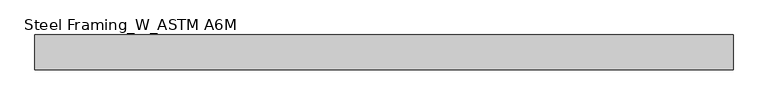
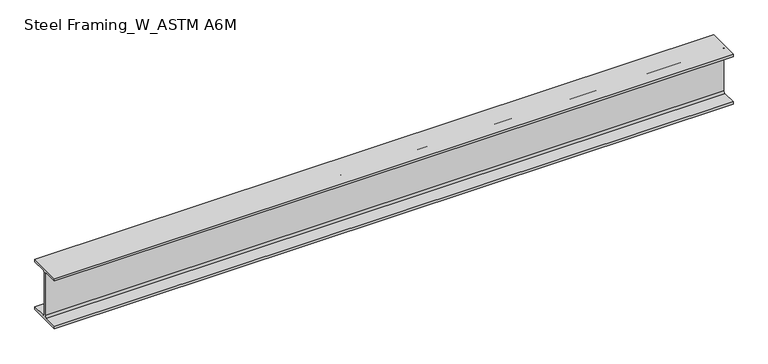
"""IFC4 building model written with IfcOpenShell, lengths in millimetres: beam geometry, Steel Framing_W_ASTM A6M : H_SB_AR_S02_W200x31.3_B6."""

from ifc_helpers import new_model, si_unit, point, frame, frame_2d, origin, place, context, project, spatial, polyline, circle_curve, trimmed, segment, composite_curve, outline, extrude, source, transform, mapped, element, save


def steel_framing_w_astm_a6m_f33feb28(model_context):
    return source(origin(), model_context, "Body", "SweptSolid", [
        extrude(outline(composite_curve([segment(polyline([(67.0, -94.8), (67.0, -105.0), (-67.0, -105.0), (-67.0, -94.8), (-10.775, -94.8)]), True, "CONTINUOUS"), segment(trimmed(circle_curve(frame_2d((-10.775, -87.2)), 7.6), [point((-10.775, -94.8))], [point((-3.175, -87.2))], True, "CARTESIAN"), True, "CONTINUOUS"), segment(polyline([(-3.175, -87.2), (-3.175, 87.2)]), True, "CONTINUOUS"), segment(trimmed(circle_curve(frame_2d((-10.775, 87.2)), 7.6), [point((-3.175, 87.2))], [point((-10.775, 94.8))], True, "CARTESIAN"), True, "CONTINUOUS"), segment(polyline([(-10.775, 94.8), (-67.0, 94.8), (-67.0, 105.0), (67.0, 105.0), (67.0, 94.8), (10.775, 94.8)]), True, "CONTINUOUS"), segment(trimmed(circle_curve(frame_2d((10.775, 87.2)), 7.6), [point((10.775, 94.8))], [point((3.175, 87.2))], True, "CARTESIAN"), True, "CONTINUOUS"), segment(polyline([(3.175, 87.2), (3.175, -87.2)]), True, "CONTINUOUS"), segment(trimmed(circle_curve(frame_2d((10.775, -87.2)), 7.6), [point((3.175, -87.2))], [point((10.775, -94.8))], True, "CARTESIAN"), True, "CONTINUOUS"), segment(polyline([(10.775, -94.8), (67.0, -94.8)]), True, "CONTINUOUS")], self_intersect=False)), frame((-1346.3, 0.0, 0.0), z_axis=(1.0, 0.0, 0.0), x_axis=(0.0, 1.0, 0.0)), (0.0, 0.0, 1.0), 2692.6),
    ])


if __name__ == "__main__":
    model = new_model("IFC4")
    model_context = context("Model", 3, world=origin())
    ifc_project = project(units=[si_unit("LENGTHUNIT", "METRE", prefix="MILLI")], contexts=[model_context])
    site = spatial("IfcSite", under=ifc_project)
    building = spatial("IfcBuilding", under=site)
    placement = place(None, origin())
    steel_framing_w_astm_a6m_shape = steel_framing_w_astm_a6m_f33feb28(model_context)
    element("IfcBeam", 1, ObjectType="Steel Framing_W_ASTM A6M : H_SB_AR_S02_W200x31.3_B6", at=placement, inside=building, context=model_context, shape_type="MappedRepresentation", body=[
        mapped(steel_framing_w_astm_a6m_shape, transform((0.0, 0.0, 0.0), x_axis=(1.0, 0.0, 0.0), y_axis=(0.0, 1.0, 0.0), z_axis=(0.0, 0.0, 1.0))),
    ])
    save(model, "model.ifc")

# Revit data of these elements
# Type "Steel Framing_W_ASTM A6M : H_SB_AR_S02_W200x31.3_B6"
#   Type Mark = "B6"
#   Section Name Key = "W8x21"
#   Width = 13.4 cm
#   Web Thickness = 0.635 cm
#   Web Fillet = 0.76 cm
#   Warping Constant = 40800.0 cm⁶
#   Torsional Moment of Inertia = 11.70 cm⁴
#   Section Area = 39.7 cm²
#   Plastic Modulus weak axis = 93.2 cm³
#   Plastic Modulus strong axis = 334.0 cm³
#   Perimeter = 0.93 m²/m
#   Nominal Weight = 31.30 kgf/m
#   Moment of Inertia weak axis = 407.00 cm⁴
#   Moment of Inertia strong axis = 3130.00 cm⁴
#   Height = 21.0 cm
#   Flange Thickness = 1.02 cm
#   Elastic Modulus weak axis = 60.8 cm³
#   Elastic Modulus strong axis = 298.0 cm³
#   Centroid Vertical = 10.5 cm
#   Centroid Horizontal = 6.7 cm
#   Length [instance default] = 1500 mm
#   Structural Material [instance default] = Steel, 45-345
#   Bolt Spacing = 0
#   Assembly Code = ""
# Element 1 (IfcBeam, "Steel Framing_W_ASTM A6M : H_SB_AR_S02_W200x31.3_B6")
#   Materials on its faces: "Steel, 45-345"
# Materials
#   "Steel, 45-345": class "Metal", colour RGB 189 187 185, transparency 0, Description = "Steel 345 MPa", Cost = 0
